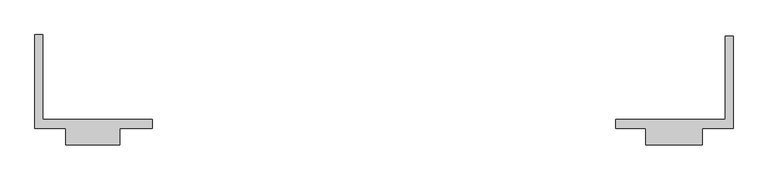
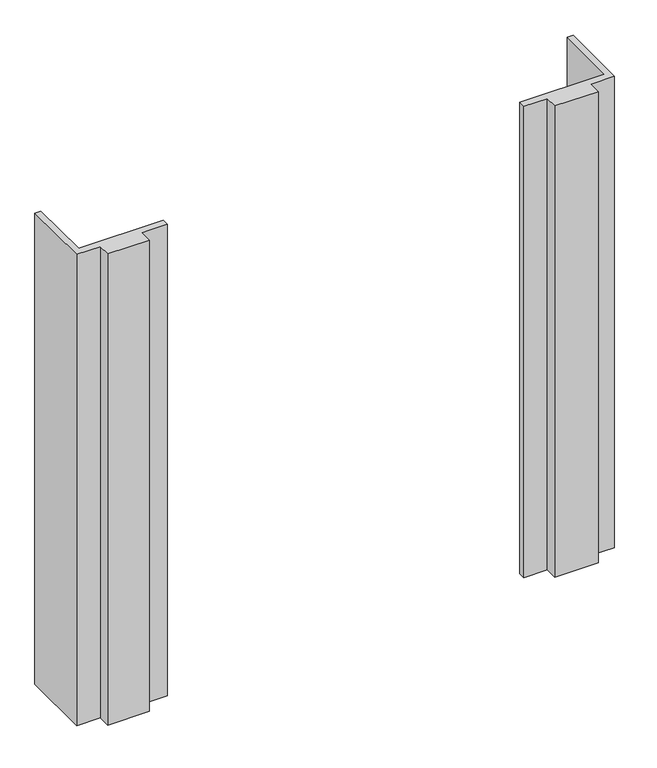
"""IFC4 building model written with IfcOpenShell, lengths in millimetres: furniture geometry, Fireplace Souround : Fireplace Souround."""

from ifc_helpers import new_model, si_unit, frame, origin, place, context, project, spatial, polyline, outline, extrude, source, transform, mapped, element, save


def furniture_11279115(model_context):
    return source(origin(), model_context, "Body", "SweptSolid", [
        extrude(outline(polyline([(133.35, 11628.4375), (133.35, 11860.2125), (152.4, 11860.2125), (152.4, 11650.6625), (423.8625, 11650.6625), (423.8625, 11628.4375), (342.8114517, 11628.4375), (342.8114517, 11587.1625), (209.55, 11587.1625), (209.55, 11628.4375), (133.35, 11628.4375)])), frame((0.0, 0.0, 177.8), z_axis=(0.0, 0.0, 1.0), x_axis=(1.0, 0.0, 0.0)), (0.0, 0.0, 1.0), 1600.2),
        extrude(outline(polyline([(1860.55, 11628.4375), (1784.35, 11628.4375), (1784.35, 11587.1625), (1644.65, 11587.1625), (1644.65, 11628.4375), (1570.0375, 11628.4375), (1570.0375, 11650.6625), (1841.5, 11650.6625), (1841.5, 11857.0375), (1860.55, 11857.0375), (1860.55, 11628.4375)])), frame((0.0, 0.0, 177.8), z_axis=(0.0, 0.0, 1.0), x_axis=(1.0, 0.0, 0.0)), (0.0, 0.0, 1.0), 1600.2),
    ])


if __name__ == "__main__":
    model = new_model("IFC4")
    model_context = context("Model", 3, world=origin())
    ifc_project = project(units=[si_unit("LENGTHUNIT", "METRE", prefix="MILLI")], contexts=[model_context])
    site = spatial("IfcSite", under=ifc_project)
    building = spatial("IfcBuilding", under=site)
    placement = place(None, origin())
    furniture_shape = furniture_11279115(model_context)
    element("IfcFurniture", 1, ObjectType="Fireplace Souround : Fireplace Souround", at=placement, inside=building, context=model_context, shape_type="MappedRepresentation", body=[
        mapped(furniture_shape, transform((0.0, 0.0, 0.0), x_axis=(1.0, 0.0, 0.0), y_axis=(0.0, 1.0, 0.0), z_axis=(0.0, 0.0, 1.0))),
    ])
    save(model, "model.ifc")

# Revit data of these elements
# Type "Fireplace Souround : Fireplace Souround"
#   COBie.Type = no
# Element 1 (IfcFurniture, "Fireplace Souround : Fireplace Souround")
#   Materials on its faces: "Trim - White"
# Materials
#   "Trim - White": class "Wood", colour RGB 255 255 255, transparency 0, Cost = 0
